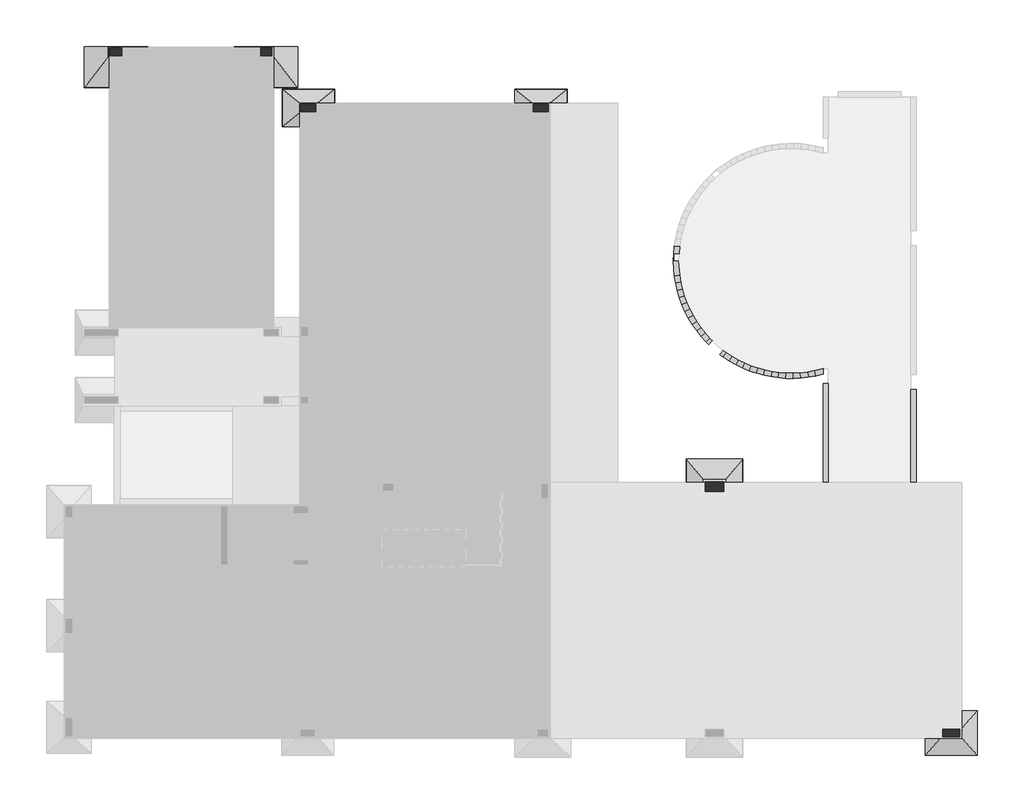
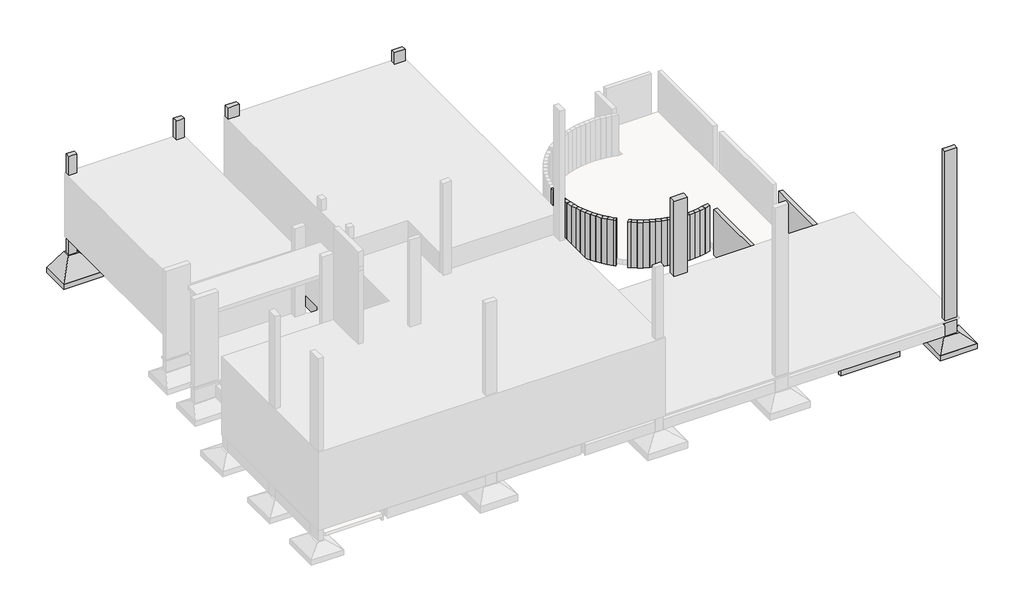
# One storey, part 3 of 4: 35 beams, 7 fasteners, 6 columns.
"""IFC4 building model written with IfcOpenShell, lengths in millimetres."""

import ifcopenshell
import ifcopenshell.guid

model = None  # the IFC model being written
_history = None  # IfcOwnerHistory: only IFC2X3 demands one
_inside = {}  # id of a spatial element -> (the spatial element, [elements in it])
_under = {}  # id of a project, library or spatial element -> (it, [spatial elements below it])
_declared = {}  # id of a project -> (the project, [libraries it declares])
_typed = {}  # id of a type object -> (the type object, [elements of that type])
_made_of = {}  # id of a material, layer set ... -> (it, [elements and type objects made of it])


def new_model(schema):
    """Start an empty IFC model of exactly this schema.

    Asked for "IFC4X3", IfcOpenShell would pick the latest addendum, in which some entities
    have other attributes; the version numbers below select the first issue.
    IFC2X3 requires an IfcOwnerHistory on every rooted entity: one is made here for all.
    """
    global model, _history
    if schema == "IFC4X3":
        model = ifcopenshell.file(schema_version=(4, 3, 0, 0))
    else:
        model = ifcopenshell.file(schema=schema)
    _inside.clear()
    _under.clear()
    _declared.clear()
    _typed.clear()
    _made_of.clear()
    _history = None
    if model.schema == "IFC2X3":
        org = make("IfcOrganization", Name="unknown")
        user = make(
            "IfcPersonAndOrganization",
            ThePerson=make("IfcPerson", FamilyName="unknown"),
            TheOrganization=org,
        )
        app = make(
            "IfcApplication",
            ApplicationDeveloper=org,
            Version="unknown",
            ApplicationFullName="unknown",
            ApplicationIdentifier="unknown",
        )
        _history = make(
            "IfcOwnerHistory",
            OwningUser=user,
            OwningApplication=app,
            ChangeAction="ADDED",
            CreationDate=0,
        )
    return model


def make(cls, **values):
    """One entity of the class cls with the attributes given. An attribute that is None is left unset."""
    return model.create_entity(
        cls, **{name: value for name, value in values.items() if value is not None}
    )


def rooted(cls, **values):
    """An entity with a GlobalId (a new one), such as an element, a storey or a relation."""
    return make(cls, GlobalId=ifcopenshell.guid.new(), OwnerHistory=_history, **values)


def si_unit(unit_type, name, prefix=None):
    """IfcSIUnit, for example si_unit("LENGTHUNIT", "METRE", prefix="MILLI")."""
    return make("IfcSIUnit", UnitType=unit_type, Prefix=prefix, Name=name)


def assignment(units):
    """IfcUnitAssignment: the units of a project."""
    return None if units is None else make("IfcUnitAssignment", Units=units)


def point(xyz):
    """IfcCartesianPoint."""
    return None if xyz is None else make("IfcCartesianPoint", Coordinates=xyz)


def direction(xyz):
    """IfcDirection."""
    return None if xyz is None else make("IfcDirection", DirectionRatios=xyz)


def frame(location, z_axis=None, x_axis=None):
    """IfcAxis2Placement3D, a coordinate frame: its origin and axes. An axis left out is left unset."""
    return make(
        "IfcAxis2Placement3D",
        Location=point(location),
        Axis=direction(z_axis),
        RefDirection=direction(x_axis),
    )


def frame_2d(location, x_axis=None):
    """IfcAxis2Placement2D, a coordinate frame in the plane: its origin and x axis."""
    return make(
        "IfcAxis2Placement2D", Location=point(location), RefDirection=direction(x_axis)
    )


def origin():
    """The frame at (0, 0, 0) with its axes left unset."""
    return frame((0.0, 0.0, 0.0))


def place(relative_to, where):
    """IfcLocalPlacement: puts the frame where relative to a parent placement (None: the world)."""
    return make(
        "IfcLocalPlacement", PlacementRelTo=relative_to, RelativePlacement=where
    )


def context(
    kind, dimensions, precision=None, world=None, true_north=None, identifier=None
):
    """IfcGeometricRepresentationContext, for example the 3D "Model" context."""
    return make(
        "IfcGeometricRepresentationContext",
        ContextIdentifier=identifier,
        ContextType=kind,
        CoordinateSpaceDimension=dimensions,
        Precision=precision,
        WorldCoordinateSystem=world,
        TrueNorth=true_north,
    )


def project(units=None, contexts=None):
    """IfcProject with its units and contexts."""
    return rooted(
        "IfcProject",
        Name="project",
        RepresentationContexts=contexts,
        UnitsInContext=assignment(units),
    )


def spatial(cls, under=None, at=None, **own):
    """A site, building, storey or space (cls), placed at a placement, below another one or the project."""
    s = rooted(cls, ObjectPlacement=at, **own)
    if under is not None:
        _under.setdefault(under.id(), (under, []))[1].append(s)
    return s


def polyline(points):
    """IfcPolyline through the points."""
    return make("IfcPolyline", Points=[point(p) for p in points])


def circle_curve(where, radius):
    """IfcCircle in the frame where."""
    return make("IfcCircle", Position=where, Radius=radius)


def trimmed(basis, trim1, trim2, sense, master):
    """IfcTrimmedCurve: the piece of a basis curve between two trims."""
    return make(
        "IfcTrimmedCurve",
        BasisCurve=basis,
        Trim1=trim1,
        Trim2=trim2,
        SenseAgreement=sense,
        MasterRepresentation=master,
    )


def segment(curve, same_sense, transition):
    """IfcCompositeCurveSegment."""
    return make(
        "IfcCompositeCurveSegment",
        Transition=transition,
        SameSense=same_sense,
        ParentCurve=curve,
    )


def composite_curve(segments, self_intersect=None):
    """IfcCompositeCurve: segments joined end to end."""
    return make("IfcCompositeCurve", Segments=segments, SelfIntersect=self_intersect)


def outline(outer, holes=None, kind="AREA"):
    """IfcArbitraryClosedProfileDef: a profile drawn as a closed curve; with holes, ...WithVoids."""
    if holes is None:
        return make("IfcArbitraryClosedProfileDef", ProfileType=kind, OuterCurve=outer)
    return make(
        "IfcArbitraryProfileDefWithVoids",
        ProfileType=kind,
        OuterCurve=outer,
        InnerCurves=holes,
    )


def extrude(swept, where, along, depth):
    """IfcExtrudedAreaSolid: the profile swept, set in the frame where, extruded along a direction by depth."""
    return make(
        "IfcExtrudedAreaSolid",
        SweptArea=swept,
        Position=where,
        ExtrudedDirection=direction(along),
        Depth=depth,
    )


def faces_of(points, faces, orient=None, outer=None):
    """IfcFace entities. A face is a list of loops; a loop is a list of indices into points, from 0.

    orient and outer hold one flag for each loop. By default every Orientation is true, the
    first loop of a face is its IfcFaceOuterBound and the others are IfcFaceBound.
    """
    made = []
    for i, loops in enumerate(faces):
        bounds = []
        for j, loop in enumerate(loops):
            is_outer = j == 0 if outer is None else outer[i][j]
            bounds.append(
                make(
                    "IfcFaceOuterBound" if is_outer else "IfcFaceBound",
                    Bound=make("IfcPolyLoop", Polygon=[points[k] for k in loop]),
                    Orientation=True if orient is None else orient[i][j],
                )
            )
        made.append(make("IfcFace", Bounds=bounds))
    return made


def faceted_brep(points, faces, orient=None, outer=None, voids=None):
    """IfcFacetedBrep: a solid bounded by flat faces; with voids (closed shells), ...WithVoids."""
    shared = [point(p) for p in points]
    hull = make("IfcClosedShell", CfsFaces=faces_of(shared, faces, orient, outer))
    if voids is None:
        return make("IfcFacetedBrep", Outer=hull)
    return make(
        "IfcFacetedBrepWithVoids",
        Outer=hull,
        Voids=[
            make(cls, CfsFaces=faces_of(shared, fs, o, b)) for cls, fs, o, b in voids
        ],
    )


def shape(context_of_items, identifier, shape_type, items):
    """IfcShapeRepresentation: the items that make up one representation, for example the "Body"."""
    return make(
        "IfcShapeRepresentation",
        ContextOfItems=context_of_items,
        RepresentationIdentifier=identifier,
        RepresentationType=shape_type,
        Items=items,
    )


def source(mapping_origin, context_of_items, identifier, shape_type, items):
    """IfcRepresentationMap: a shape defined once, which mapped items show again and again."""
    return make(
        "IfcRepresentationMap",
        MappingOrigin=mapping_origin,
        MappedRepresentation=shape(context_of_items, identifier, shape_type, items),
    )


def transform(
    local_origin,
    x_axis=None,
    y_axis=None,
    z_axis=None,
    scale=None,
    scale2=None,
    scale3=None,
    uniform=True,
):
    """IfcCartesianTransformationOperator3D, or its non-uniform kind. x_axis, y_axis, z_axis: its Axis1, 2, 3."""
    if uniform:
        return make(
            "IfcCartesianTransformationOperator3D",
            Axis1=direction(x_axis),
            Axis2=direction(y_axis),
            LocalOrigin=point(local_origin),
            Scale=scale,
            Axis3=direction(z_axis),
        )
    return make(
        "IfcCartesianTransformationOperator3DnonUniform",
        Axis1=direction(x_axis),
        Axis2=direction(y_axis),
        LocalOrigin=point(local_origin),
        Scale=scale,
        Axis3=direction(z_axis),
        Scale2=scale2,
        Scale3=scale3,
    )


def mapped(mapping_source, mapping_target):
    """IfcMappedItem: shows the shape of a source again, moved by a transform."""
    return make(
        "IfcMappedItem", MappingSource=mapping_source, MappingTarget=mapping_target
    )


def made_of(thing, what):
    """Note that an element or type object is made of a material, layer set ...; save() writes the relation."""
    if what is not None:
        _made_of.setdefault(what.id(), (what, []))[1].append(thing)
    return thing


def element(
    cls,
    number,
    at=None,
    inside=None,
    cuts=None,
    type_object=None,
    material=None,
    context=None,
    identifier="Body",
    shape_type=None,
    held_by="IfcProductDefinitionShape",
    body=None,
    shapes=None,
    **own,
):
    """One element of the class cls, such as IfcWall. Its Tag is "e" and its number.

    at: its placement. inside: the storey or other place that contains it. cuts: it is an
    opening in that element (IfcRelVoidsElement). A single representation is given by context,
    identifier, shape_type and body (its items); several are given by shapes. held_by: the class
    of the entity that holds the representations. save() writes the other relations.
    """
    e = rooted(cls, Tag="e%d" % number, ObjectPlacement=at, **own)
    if body is not None:
        shapes = [shape(context, identifier, shape_type, body)]
    if shapes is not None:
        e.Representation = make(held_by, Representations=shapes)
    if inside is not None:
        _inside.setdefault(inside.id(), (inside, []))[1].append(e)
    if cuts is not None:
        rooted(
            "IfcRelVoidsElement", RelatingBuildingElement=cuts, RelatedOpeningElement=e
        )
    if type_object is not None:
        _typed.setdefault(type_object.id(), (type_object, []))[1].append(e)
    return made_of(e, material)


def aggregate(whole, parts):
    """IfcRelAggregates: a whole, such as a stair, and the parts it consists of."""
    return rooted("IfcRelAggregates", RelatingObject=whole, RelatedObjects=parts)


def save(model, path):
    """Write the relations noted so far, then the file.

    IfcRelAggregates (storeys below a building ...), IfcRelContainedInSpatialStructure (elements
    in a storey), IfcRelDefinesByType, IfcRelAssociatesMaterial and IfcRelDeclares: one each for
    every whole, place, type object, material and project.
    """
    for whole, parts in _under.values():
        aggregate(whole, parts)
    for where, things in _inside.values():
        rooted(
            "IfcRelContainedInSpatialStructure",
            RelatedElements=things,
            RelatingStructure=where,
        )
    for kind, things in _typed.values():
        rooted("IfcRelDefinesByType", RelatedObjects=things, RelatingType=kind)
    for what, things in _made_of.values():
        rooted("IfcRelAssociatesMaterial", RelatedObjects=things, RelatingMaterial=what)
    for by, libraries in _declared.values():
        rooted("IfcRelDeclares", RelatingContext=by, RelatedDefinitions=libraries)
    model.write(path)


def tqs_viga_retangular_19_0_x_30_0_29604a85(model_context):
    return source(origin(), model_context, "Body", "SweptSolid", [
        extrude(outline(polyline([(1809.0, 95.0), (1809.0, -95.0), (-1809.0, -95.0), (-1809.0, 95.0), (1809.0, 95.0)])), frame((0.0, 0.0, -150.0), z_axis=(0.0, 0.0, 1.0), x_axis=(1.0, 0.0, 0.0)), (0.0, 0.0, 1.0), 300.0),
    ])


def s1_ccae0304(model_context):
    return source(origin(), model_context, "Body", "SolidModel", [
        faceted_brep([(-460.0, 0.0, 0.0), (-750.0, 0.0, 0.0), (-750.0, -400.0, 0.0), (-460.0, -400.0, 0.0), (350.0, 650.0, -400.0), (350.0, -1050.0, -400.0), (-750.0, -1050.0, -400.0), (-750.0, 650.0, -400.0)], [[[0, 1, 2, 3]], [[4, 5, 6, 7]], [[4, 7, 1, 0]], [[7, 6, 2, 1]], [[6, 5, 3, 2]], [[5, 4, 0, 3]]]),
        extrude(outline(polyline([(350.0, 650.0), (350.0, -1050.0), (-750.0, -1050.0), (-750.0, 650.0), (350.0, 650.0)])), frame((0.0, 0.0, -600.0), z_axis=(0.0, 0.0, 1.0), x_axis=(1.0, 0.0, 0.0)), (0.0, 0.0, 1.0), 200.0),
    ])


def s12_1e6d1b45(model_context):
    return source(origin(), model_context, "Body", "SolidModel", [
        faceted_brep([(-55.0, 50.0, 0.0), (-345.0, 50.0, 0.0), (-345.0, -450.0, 0.0), (-55.0, -450.0, 0.0), (550.0, 550.0, -350.0), (550.0, -950.0, -350.0), (-950.0, -950.0, -350.0), (-950.0, 550.0, -350.0)], [[[0, 1, 2, 3]], [[4, 5, 6, 7]], [[4, 7, 1, 0]], [[7, 6, 2, 1]], [[6, 5, 3, 2]], [[5, 4, 0, 3]]]),
        extrude(outline(polyline([(550.0, 550.0), (550.0, -950.0), (-950.0, -950.0), (-950.0, 550.0), (550.0, 550.0)])), frame((0.0, 0.0, -600.0), z_axis=(0.0, 0.0, 1.0), x_axis=(1.0, 0.0, 0.0)), (0.0, 0.0, 1.0), 250.0),
    ])


def s13_7eae1afe(model_context):
    return source(origin(), model_context, "Body", "SolidModel", [
        faceted_brep([(-5.0, 100.0, 0.0), (-395.0, 100.0, 0.0), (-395.0, -500.0, 0.0), (-5.0, -500.0, 0.0), (550.0, 550.0, -300.0), (550.0, -950.0, -300.0), (-950.0, -950.0, -300.0), (-950.0, 550.0, -300.0)], [[[0, 1, 2, 3]], [[4, 5, 6, 7]], [[4, 7, 1, 0]], [[7, 6, 2, 1]], [[6, 5, 3, 2]], [[5, 4, 0, 3]]]),
        extrude(outline(polyline([(550.0, 550.0), (550.0, -950.0), (-950.0, -950.0), (-950.0, 550.0), (550.0, 550.0)])), frame((0.0, 0.0, -500.0), z_axis=(0.0, 0.0, 1.0), x_axis=(1.0, 0.0, 0.0)), (0.0, 0.0, 1.0), 200.0),
    ])


def s20_c409a0c5(model_context):
    return source(origin(), model_context, "Body", "SolidModel", [
        faceted_brep([(-55.0, 100.0, 0.0), (-345.0, 100.0, 0.0), (-345.0, -500.0, 0.0), (-55.0, -500.0, 0.0), (400.0, 500.0, -300.0), (400.0, -900.0, -300.0), (-800.0, -900.0, -300.0), (-800.0, 500.0, -300.0)], [[[0, 1, 2, 3]], [[4, 5, 6, 7]], [[4, 7, 1, 0]], [[7, 6, 2, 1]], [[6, 5, 3, 2]], [[5, 4, 0, 3]]]),
        extrude(outline(polyline([(400.0, 500.0), (400.0, -900.0), (-800.0, -900.0), (-800.0, 500.0), (400.0, 500.0)])), frame((0.0, 0.0, -500.0), z_axis=(0.0, 0.0, 1.0), x_axis=(1.0, 0.0, 0.0)), (0.0, 0.0, 1.0), 200.0),
    ])


def s3_fc183e28(model_context):
    return source(origin(), model_context, "Body", "SolidModel", [
        faceted_brep([(-55.0, 50.0, 0.0), (-345.0, 50.0, 0.0), (-345.0, -450.0, 0.0), (-55.0, -450.0, 0.0), (300.0, 500.0, -300.0), (300.0, -900.0, -300.0), (-700.0, -900.0, -300.0), (-700.0, 500.0, -300.0)], [[[0, 1, 2, 3]], [[4, 5, 6, 7]], [[4, 7, 1, 0]], [[7, 6, 2, 1]], [[6, 5, 3, 2]], [[5, 4, 0, 3]]]),
        extrude(outline(polyline([(300.0, 500.0), (300.0, -900.0), (-700.0, -900.0), (-700.0, 500.0), (300.0, 500.0)])), frame((0.0, 0.0, -500.0), z_axis=(0.0, 0.0, 1.0), x_axis=(1.0, 0.0, 0.0)), (0.0, 0.0, 1.0), 200.0),
    ])


model = new_model("IFC4")

# Units and contexts
model_context = context("Model", 3, world=origin())
ifc_project = project(units=[si_unit("LENGTHUNIT", "METRE", prefix="MILLI")], contexts=[model_context])

# Site, building, storey
site = spatial("IfcSite", under=ifc_project)
building = spatial("IfcBuilding", under=site)
storey = spatial("IfcBuildingStorey", under=building, Name="PAVIMENTO TÉRREO", Elevation=500.0)

# Beams
placement = place(None, origin())
element("IfcBeam", 1, ObjectType="TQS - Viga retangular : 14.0 x 180.0", at=placement, inside=storey, context=model_context, shape_type="Brep", body=[
    faceted_brep([(9682.718693, -9679.5699847, 350.0), (9682.718693, -9539.5699847, 350.0), (7474.718693, -9539.5699847, 350.0), (7474.718693, -9679.5699847, 350.0), (9682.718693, -9679.5699847, -1450.0), (7474.718693, -9679.5699847, -1450.0), (9682.718693, -9539.5699847, -1450.0), (7474.718693, -9539.5699847, -1450.0), (9682.718693, -9539.5699847, -1250.0), (7474.718693, -9539.5699847, -1250.0)], [[[0, 1, 2, 3]], [[4, 0, 3, 5]], [[6, 4, 5, 7]], [[1, 8, 6, 7, 9, 2]], [[2, 9, 7, 5, 3]], [[1, 0, 4, 6, 8]]]),
])
element("IfcBeam", 2, ObjectType="TQS - Viga retangular : 14.0 x 180.0", at=placement, inside=storey, context=model_context, shape_type="Brep", body=[
    faceted_brep([(7474.718693, -1696.0936198, 350.0), (7334.718693, -1696.0936198, 350.0), (7334.718693, -5230.1494451, 350.0), (7474.718693, -5230.1494451, 350.0), (7474.718693, -5230.1494451, -1250.0), (7474.718693, -5230.1494451, -1450.0), (7474.718693, -1696.0936198, -1450.0), (7474.718693, -1696.0936198, -1250.0), (7334.718693, -1696.0936198, -1450.0), (7334.718693, -5230.1494451, -1450.0)], [[[0, 1, 2, 3]], [[0, 3, 4, 5, 6, 7]], [[8, 6, 5, 9]], [[1, 8, 9, 2]], [[1, 0, 7, 6, 8]], [[3, 2, 9, 5, 4]]]),
    faceted_brep([(7334.718693, -5630.1494451, 350.0), (7474.718693, -5630.1494451, 350.0), (7474.718693, -5630.1494451, -1250.0), (7474.718693, -5630.1494451, -1450.0), (7334.718693, -5630.1494451, -1450.0), (7334.718693, -9279.5699847, 350.0), (7474.718693, -9279.5699847, 350.0), (7474.718693, -9279.5699847, -1250.0), (7474.718693, -9279.5699847, -1450.0), (7334.718693, -9279.5699847, -1450.0)], [[[0, 1, 2, 3, 4]], [[1, 0, 5, 6]], [[1, 6, 7, 8, 3, 2]], [[4, 3, 8, 9]], [[0, 4, 9, 5]], [[6, 5, 9, 8, 7]]]),
])
element("IfcBeam", 3, ObjectType="TQS - Viga retangular : 14.0 x 180.0", at=placement, inside=storey, context=model_context, shape_type="Brep", body=[
    faceted_brep([(7334.718693, -1296.0936198, 350.0), (7106.1277936, -1352.3610531, 350.0), (7135.2990206, -1489.35947, 350.0), (7334.718693, -1440.2725066, 350.0), (7334.718693, -1296.0936198, -1250.0), (7334.718693, -1296.0936198, -1450.0), (7106.1277936, -1352.3610531, -1450.0), (7106.1277936, -1352.3610531, -1250.0), (7334.718693, -1440.2725066, -1450.0), (7135.2990206, -1489.35947, -1450.0)], [[[0, 1, 2, 3]], [[1, 0, 4, 5, 6, 7]], [[6, 5, 8, 9]], [[3, 2, 9, 8]], [[0, 3, 8, 5, 4]], [[2, 1, 7, 6, 9]]]),
])
element("IfcBeam", 4, ObjectType="TQS - Viga retangular : 14.0 x 180.0", at=placement, inside=storey, context=model_context, shape_type="Brep", body=[
    faceted_brep([(6938.2242767, -1524.8638101, 350.0), (7135.2990206, -1489.35947, 350.0), (7106.1277936, -1352.3610531, 350.0), (6917.7849868, -1386.2922761, 350.0), (7106.1277936, -1352.3610531, -1250.0), (7106.1277936, -1352.3610531, -1450.0), (6917.7849868, -1386.2922761, -1450.0), (6917.7849868, -1386.2922761, -1250.0), (7135.2990206, -1489.35947, -1450.0), (6938.2242767, -1524.8638101, -1450.0)], [[[0, 1, 2, 3]], [[3, 2, 4, 5, 6, 7]], [[6, 5, 8, 9]], [[1, 0, 9, 8]], [[1, 8, 5, 4, 2]], [[0, 3, 7, 6, 9]]]),
])
element("IfcBeam", 5, ObjectType="TQS - Viga retangular : 14.0 x 180.0", at=placement, inside=storey, context=model_context, shape_type="Brep", body=[
    faceted_brep([(6739.2913899, -1547.770563, 350.0), (6938.2242767, -1524.8638101, 350.0), (6917.7849868, -1386.2922761, 350.0), (6727.7008432, -1408.1801126, 350.0), (6917.7849868, -1386.2922761, -1250.0), (6917.7849868, -1386.2922761, -1450.0), (6727.7008432, -1408.1801126, -1450.0), (6727.7008432, -1408.1801126, -1250.0), (6938.2242767, -1524.8638101, -1450.0), (6739.2913899, -1547.770563, -1450.0)], [[[0, 1, 2, 3]], [[3, 2, 4, 5, 6, 7]], [[6, 5, 8, 9]], [[1, 0, 9, 8]], [[1, 8, 5, 4, 2]], [[0, 3, 7, 6, 9]]]),
])
element("IfcBeam", 6, ObjectType="TQS - Viga retangular : 14.0 x 180.0", at=placement, inside=storey, context=model_context, shape_type="Brep", body=[
    faceted_brep([(6539.3048029, -1557.9870986, 350.0), (6739.2913899, -1547.770563, 350.0), (6727.7008432, -1408.1801126, 350.0), (6536.6098693, -1417.942206, 350.0), (6727.7008432, -1408.1801126, -1250.0), (6727.7008432, -1408.1801126, -1450.0), (6536.6098693, -1417.942206, -1450.0), (6536.6098693, -1417.942206, -1250.0), (6739.2913899, -1547.770563, -1450.0), (6539.3048029, -1557.9870986, -1450.0)], [[[0, 1, 2, 3]], [[3, 2, 4, 5, 6, 7]], [[6, 5, 8, 9]], [[1, 0, 9, 8]], [[1, 8, 5, 4, 2]], [[0, 3, 7, 6, 9]]]),
])
element("IfcBeam", 7, ObjectType="TQS - Viga retangular : 14.0 x 180.0", at=placement, inside=storey, context=model_context, shape_type="Brep", body=[
    faceted_brep([(6339.0732182, -1555.4721035, 350.0), (6539.3048029, -1557.9870986, 350.0), (6536.6098693, -1417.942206, 350.0), (6345.2847953, -1415.5390805, 350.0), (6536.6098693, -1417.942206, -1250.0), (6536.6098693, -1417.942206, -1450.0), (6345.2847953, -1415.5390805, -1450.0), (6345.2847953, -1415.5390805, -1250.0), (6539.3048029, -1557.9870986, -1450.0), (6339.0732182, -1555.4721035, -1450.0)], [[[0, 1, 2, 3]], [[3, 2, 4, 5, 6, 7]], [[6, 5, 8, 9]], [[1, 0, 9, 8]], [[1, 8, 5, 4, 2]], [[0, 3, 7, 6, 9]]]),
])
element("IfcBeam", 8, ObjectType="TQS - Viga retangular : 14.0 x 180.0", at=placement, inside=storey, context=model_context, shape_type="Brep", body=[
    faceted_brep([(6139.4063301, -1540.2357477, 350.0), (6339.0732182, -1555.4721035, 350.0), (6345.2847953, -1415.5390805, 350.0), (6154.4732894, -1400.978469, 350.0), (6345.2847953, -1415.5390805, -1250.0), (6345.2847953, -1415.5390805, -1450.0), (6154.4732894, -1400.978469, -1450.0), (6154.4732894, -1400.978469, -1250.0), (6339.0732182, -1555.4721035, -1450.0), (6139.4063301, -1540.2357477, -1450.0)], [[[0, 1, 2, 3]], [[3, 2, 4, 5, 6, 7]], [[6, 5, 8, 9]], [[1, 0, 9, 8]], [[1, 8, 5, 4, 2]], [[0, 3, 7, 6, 9]]]),
])
element("IfcBeam", 9, ObjectType="TQS - Viga retangular : 14.0 x 180.0", at=placement, inside=storey, context=model_context, shape_type="Brep", body=[
    faceted_brep([(5942.253541, -1512.5751442, 350.0), (6139.4063301, -1540.2357477, 350.0), (6154.4732894, -1400.978469, 350.0), (5966.1413215, -1374.5554297, 350.0), (6154.4732894, -1400.978469, -1250.0), (6154.4732894, -1400.978469, -1450.0), (5966.1413215, -1374.5554297, -1450.0), (5966.1413215, -1374.5554297, -1250.0), (6139.4063301, -1540.2357477, -1450.0), (5942.253541, -1512.5751442, -1450.0)], [[[0, 1, 2, 3]], [[3, 2, 4, 5, 6, 7]], [[6, 5, 8, 9]], [[1, 0, 9, 8]], [[1, 8, 5, 4, 2]], [[0, 3, 7, 6, 9]]]),
])
element("IfcBeam", 10, ObjectType="TQS - Viga retangular : 14.0 x 180.0", at=placement, inside=storey, context=model_context, shape_type="Brep", body=[
    faceted_brep([(5746.1327296, -1472.1320983, 350.0), (5942.253541, -1512.5751442, 350.0), (5966.1413215, -1374.5554297, 350.0), (5778.7697179, -1335.9166013, 350.0), (5966.1413215, -1374.5554297, -1250.0), (5966.1413215, -1374.5554297, -1450.0), (5778.7697179, -1335.9166013, -1450.0), (5778.7697179, -1335.9166013, -1250.0), (5942.253541, -1512.5751442, -1450.0), (5746.1327296, -1472.1320983, -1450.0)], [[[0, 1, 2, 3]], [[3, 2, 4, 5, 6, 7]], [[6, 5, 8, 9]], [[1, 0, 9, 8]], [[1, 8, 5, 4, 2]], [[0, 3, 7, 6, 9]]]),
])
element("IfcBeam", 11, ObjectType="TQS - Viga retangular : 14.0 x 180.0", at=placement, inside=storey, context=model_context, shape_type="Brep", body=[
    faceted_brep([(5552.9789583, -1419.3056534, 350.0), (5746.1327296, -1472.1320983, 350.0), (5778.7697179, -1335.9166013, 350.0), (5594.2076289, -1285.4399321, 350.0), (5778.7697179, -1335.9166013, -1250.0), (5778.7697179, -1335.9166013, -1450.0), (5594.2076289, -1285.4399321, -1450.0), (5594.2076289, -1285.4399321, -1250.0), (5746.1327296, -1472.1320983, -1450.0), (5552.9789583, -1419.3056534, -1450.0)], [[[0, 1, 2, 3]], [[3, 2, 4, 5, 6, 7]], [[6, 5, 8, 9]], [[1, 0, 9, 8]], [[1, 8, 5, 4, 2]], [[0, 3, 7, 6, 9]]]),
])
element("IfcBeam", 12, ObjectType="TQS - Viga retangular : 14.0 x 180.0", at=placement, inside=storey, context=model_context, shape_type="Brep", body=[
    faceted_brep([(5363.9986658, -1354.4553965, 350.0), (5552.9789583, -1419.3056534, 350.0), (5594.2076289, -1285.4399321, 350.0), (5413.6522985, -1223.4807754, 350.0), (5594.2076289, -1285.4399321, -1250.0), (5594.2076289, -1285.4399321, -1450.0), (5413.6522985, -1223.4807754, -1450.0), (5413.6522985, -1223.4807754, -1250.0), (5552.9789583, -1419.3056534, -1450.0), (5363.9986658, -1354.4553965, -1450.0)], [[[0, 1, 2, 3]], [[3, 2, 4, 5, 6, 7]], [[6, 5, 8, 9]], [[1, 0, 9, 8]], [[1, 8, 5, 4, 2]], [[0, 3, 7, 6, 9]]]),
])
element("IfcBeam", 13, ObjectType="TQS - Viga retangular : 14.0 x 180.0", at=placement, inside=storey, context=model_context, shape_type="Brep", body=[
    faceted_brep([(5179.1069104, -1277.5521698, 350.0), (5363.9986658, -1354.4553965, 350.0), (5413.6522985, -1223.4807754, 350.0), (5236.9847165, -1149.9982825, 350.0), (5413.6522985, -1223.4807754, -1250.0), (5413.6522985, -1223.4807754, -1450.0), (5236.9847165, -1149.9982825, -1450.0), (5236.9847165, -1149.9982825, -1250.0), (5363.9986658, -1354.4553965, -1450.0), (5179.1069104, -1277.5521698, -1450.0)], [[[0, 1, 2, 3]], [[3, 2, 4, 5, 6, 7]], [[6, 5, 8, 9]], [[1, 0, 9, 8]], [[1, 8, 5, 4, 2]], [[0, 3, 7, 6, 9]]]),
])
element("IfcBeam", 14, ObjectType="TQS - Viga retangular : 14.0 x 180.0", at=placement, inside=storey, context=model_context, shape_type="Brep", body=[
    faceted_brep([(4999.4769736, -1189.0530269, 350.0), (5179.1069104, -1277.5521698, 350.0), (5236.9847165, -1149.9982825, 350.0), (5065.344906, -1065.4356735, 350.0), (5236.9847165, -1149.9982825, -1250.0), (5236.9847165, -1149.9982825, -1450.0), (5065.344906, -1065.4356735, -1450.0), (5065.344906, -1065.4356735, -1250.0), (5179.1069104, -1277.5521698, -1450.0), (4999.4769736, -1189.0530269, -1450.0)], [[[0, 1, 2, 3]], [[3, 2, 4, 5, 6, 7]], [[6, 5, 8, 9]], [[1, 0, 9, 8]], [[1, 8, 5, 4, 2]], [[0, 3, 7, 6, 9]]]),
])
element("IfcBeam", 15, ObjectType="TQS - Viga retangular : 14.0 x 180.0", at=placement, inside=storey, context=model_context, shape_type="Brep", body=[
    faceted_brep([(4825.8347061, -1089.3155581, 350.0), (4999.4769736, -1189.0530269, 350.0), (5065.344906, -1065.4356735, 350.0), (4899.4264221, -970.1346281, 350.0), (5065.344906, -1065.4356735, -1250.0), (5065.344906, -1065.4356735, -1450.0), (4899.4264221, -970.1346281, -1450.0), (4899.4264221, -970.1346281, -1250.0), (4999.4769736, -1189.0530269, -1450.0), (4825.8347061, -1089.3155581, -1450.0)], [[[0, 1, 2, 3]], [[3, 2, 4, 5, 6, 7]], [[6, 5, 8, 9]], [[1, 0, 9, 8]], [[1, 8, 5, 4, 2]], [[0, 3, 7, 6, 9]]]),
])
element("IfcBeam", 16, ObjectType="TQS - Viga retangular : 14.0 x 180.0", at=placement, inside=storey, context=model_context, shape_type="Brep", body=[
    faceted_brep([(4659.7082838, -979.2900143, 350.0), (4825.8347061, -1089.3155581, 350.0), (4899.4264221, -970.1346281, 350.0), (4740.8701617, -865.1228032, 350.0), (4899.4264221, -970.1346281, -1250.0), (4899.4264221, -970.1346281, -1450.0), (4740.8701617, -865.1228032, -1450.0), (4740.8701617, -865.1228032, -1250.0), (4825.8347061, -1089.3155581, -1450.0), (4659.7082838, -979.2900143, -1450.0)], [[[0, 1, 2, 3]], [[3, 2, 4, 5, 6, 7]], [[6, 5, 8, 9]], [[1, 0, 9, 8]], [[1, 8, 5, 4, 2]], [[0, 3, 7, 6, 9]]]),
])
element("IfcBeam", 17, ObjectType="TQS - Viga retangular : 14.0 x 180.0", at=placement, inside=storey, context=model_context, shape_type="Brep", body=[
    faceted_brep([(4571.9800682, -912.4546637, 350.0), (4659.7082838, -979.2900143, 350.0), (4740.8701617, -865.1228032, 350.0), (4665.976342, -808.0652799, 350.0), (4740.8701617, -865.1228032, -1250.0), (4740.8701617, -865.1228032, -1450.0), (4665.976342, -808.0652799, -1450.0), (4665.976342, -808.0652799, -1250.0), (4659.7082838, -979.2900143, -1450.0), (4571.9800682, -912.4546637, -1450.0)], [[[0, 1, 2, 3]], [[3, 2, 4, 5, 6, 7]], [[8, 9, 6, 5]], [[1, 0, 9, 8]], [[0, 3, 7, 6, 9]], [[1, 8, 5, 4, 2]]]),
])
element("IfcBeam", 18, ObjectType="TQS - Viga retangular : 14.0 x 180.0", at=placement, inside=storey, context=model_context, shape_type="Brep", body=[
    faceted_brep([(4206.3905749, -587.9275531, 350.0), (4270.2869357, -650.1191423, 350.0), (4367.9344995, -549.7949015, 350.0), (4307.4254093, -490.9002096, 350.0), (4367.9344995, -549.7949015, -1450.0), (4362.9503182, -544.9436994, -1450.0), (4307.4254093, -490.9002096, -1450.0), (4307.4254093, -490.9002096, -1250.0), (4270.2869357, -650.1191423, -1450.0), (4206.3905749, -587.9275531, -1450.0)], [[[0, 1, 2, 3]], [[3, 2, 4, 5, 6, 7]], [[8, 9, 6, 5, 4]], [[1, 0, 9, 8]], [[1, 8, 4, 2]], [[0, 3, 7, 6, 9]]]),
])
element("IfcBeam", 19, ObjectType="TQS - Viga retangular : 14.0 x 180.0", at=placement, inside=storey, context=model_context, shape_type="Brep", body=[
    faceted_brep([(4072.6403676, -438.8977092, 350.0), (4206.3905749, -587.9275531, 350.0), (4307.4254093, -490.9002096, 350.0), (4179.8070625, -348.7027306, 350.0), (4307.4254093, -490.9002096, -1250.0), (4307.4254093, -490.9002096, -1450.0), (4179.8070625, -348.7027306, -1450.0), (4179.8070625, -348.7027306, -1250.0), (4206.3905749, -587.9275531, -1450.0), (4072.6403676, -438.8977092, -1450.0)], [[[0, 1, 2, 3]], [[3, 2, 4, 5, 6, 7]], [[6, 5, 8, 9]], [[1, 0, 9, 8]], [[1, 8, 5, 4, 2]], [[0, 3, 7, 6, 9]]]),
])
element("IfcBeam", 20, ObjectType="TQS - Viga retangular : 14.0 x 180.0", at=placement, inside=storey, context=model_context, shape_type="Brep", body=[
    faceted_brep([(3949.2502321, -282.451126, 350.0), (4072.6403676, -438.8977092, 350.0), (4179.8070625, -348.7027306, 350.0), (4061.9329165, -199.2498808, 350.0), (4179.8070625, -348.7027306, -1250.0), (4179.8070625, -348.7027306, -1450.0), (4061.9329165, -199.2498808, -1450.0), (4061.9329165, -199.2498808, -1250.0), (4072.6403676, -438.8977092, -1450.0), (3949.2502321, -282.451126, -1450.0)], [[[0, 1, 2, 3]], [[3, 2, 4, 5, 6, 7]], [[6, 5, 8, 9]], [[1, 0, 9, 8]], [[1, 8, 5, 4, 2]], [[0, 3, 7, 6, 9]]]),
])
element("IfcBeam", 21, ObjectType="TQS - Viga retangular : 14.0 x 180.0", at=placement, inside=storey, context=model_context, shape_type="Brep", body=[
    faceted_brep([(3835.4866089, -117.6577696, 350.0), (3949.2502321, -282.451126, 350.0), (4061.9329165, -199.2498808, 350.0), (3953.2296156, -41.7867013, 350.0), (4061.9329165, -199.2498808, -1250.0), (4061.9329165, -199.2498808, -1450.0), (3953.2296156, -41.7867013, -1450.0), (3953.2296156, -41.7867013, -1250.0), (3949.2502321, -282.451126, -1450.0), (3835.4866089, -117.6577696, -1450.0)], [[[0, 1, 2, 3]], [[3, 2, 4, 5, 6, 7]], [[6, 5, 8, 9]], [[1, 0, 9, 8]], [[1, 8, 5, 4, 2]], [[0, 3, 7, 6, 9]]]),
])
element("IfcBeam", 22, ObjectType="TQS - Viga retangular : 14.0 x 180.0", at=placement, inside=storey, context=model_context, shape_type="Brep", body=[
    faceted_brep([(3732.4270441, 54.0330523, 350.0), (3835.4866089, -117.6577696, 350.0), (3953.2296156, -41.7867013, 350.0), (3854.7542482, 122.2671329, 350.0), (3953.2296156, -41.7867013, -1250.0), (3953.2296156, -41.7867013, -1450.0), (3854.7542482, 122.2671329, -1450.0), (3854.7542482, 122.2671329, -1250.0), (3835.4866089, -117.6577696, -1450.0), (3732.4270441, 54.0330523, -1450.0)], [[[0, 1, 2, 3]], [[3, 2, 4, 5, 6, 7]], [[6, 5, 8, 9]], [[1, 0, 9, 8]], [[1, 8, 5, 4, 2]], [[0, 3, 7, 6, 9]]]),
])
element("IfcBeam", 23, ObjectType="TQS - Viga retangular : 14.0 x 180.0", at=placement, inside=storey, context=model_context, shape_type="Brep", body=[
    faceted_brep([(3640.48809, 231.9274426, 350.0), (3732.4270441, 54.0330523, 350.0), (3854.7542482, 122.2671329, 350.0), (3766.9048318, 292.2486007, 350.0), (3854.7542482, 122.2671329, -1250.0), (3854.7542482, 122.2671329, -1450.0), (3766.9048318, 292.2486007, -1450.0), (3766.9048318, 292.2486007, -1250.0), (3732.4270441, 54.0330523, -1450.0), (3640.48809, 231.9274426, -1450.0)], [[[0, 1, 2, 3]], [[3, 2, 4, 5, 6, 7]], [[6, 5, 8, 9]], [[1, 0, 9, 8]], [[1, 8, 5, 4, 2]], [[0, 3, 7, 6, 9]]]),
])
element("IfcBeam", 24, ObjectType="TQS - Viga retangular : 14.0 x 180.0", at=placement, inside=storey, context=model_context, shape_type="Brep", body=[
    faceted_brep([(3560.3661231, 414.5663391, 350.0), (3640.48809, 231.9274426, 350.0), (3766.9048318, 292.2486007, 350.0), (3690.3611932, 466.7306588, 350.0), (3766.9048318, 292.2486007, -1250.0), (3766.9048318, 292.2486007, -1450.0), (3690.3611932, 466.7306588, -1450.0), (3690.3611932, 466.7306588, -1250.0), (3640.48809, 231.9274426, -1450.0), (3560.3661231, 414.5663391, -1450.0)], [[[0, 1, 2, 3]], [[3, 2, 4, 5, 6, 7]], [[6, 5, 8, 9]], [[1, 0, 9, 8]], [[1, 8, 5, 4, 2]], [[0, 3, 7, 6, 9]]]),
])
element("IfcBeam", 25, ObjectType="TQS - Viga retangular : 14.0 x 180.0", at=placement, inside=storey, context=model_context, shape_type="Brep", body=[
    faceted_brep([(3491.737855, 602.6864416, 350.0), (3560.3661231, 414.5663391, 350.0), (3690.3611932, 466.7306588, 350.0), (3624.7902852, 646.4700908, 350.0), (3690.3611932, 466.7306588, -1250.0), (3690.3611932, 466.7306588, -1450.0), (3624.7902852, 646.4700908, -1450.0), (3624.7902852, 646.4700908, -1250.0), (3560.3661231, 414.5663391, -1450.0), (3491.737855, 602.6864416, -1450.0)], [[[0, 1, 2, 3]], [[3, 2, 4, 5, 6, 7]], [[6, 5, 8, 9]], [[1, 0, 9, 8]], [[1, 8, 5, 4, 2]], [[0, 3, 7, 6, 9]]]),
])
element("IfcBeam", 26, ObjectType="TQS - Viga retangular : 14.0 x 180.0", at=placement, inside=storey, context=model_context, shape_type="Brep", body=[
    faceted_brep([(3435.4159463, 794.2099051, 350.0), (3491.737855, 602.6864416, 350.0), (3624.7902852, 646.4700908, 350.0), (3570.9813422, 829.4481782, 350.0), (3624.7902852, 646.4700908, -1250.0), (3624.7902852, 646.4700908, -1450.0), (3570.9813422, 829.4481782, -1450.0), (3570.9813422, 829.4481782, -1250.0), (3491.737855, 602.6864416, -1450.0), (3435.4159463, 794.2099051, -1450.0)], [[[0, 1, 2, 3]], [[3, 2, 4, 5, 6, 7]], [[6, 5, 8, 9]], [[1, 0, 9, 8]], [[1, 8, 5, 4, 2]], [[0, 3, 7, 6, 9]]]),
])
element("IfcBeam", 27, ObjectType="TQS - Viga retangular : 14.0 x 180.0", at=placement, inside=storey, context=model_context, shape_type="Brep", body=[
    faceted_brep([(3391.2071159, 989.5163089, 350.0), (3435.4159463, 794.2099051, 350.0), (3570.9813422, 829.4481782, 350.0), (3528.735935, 1016.0805429, 350.0), (3570.9813422, 829.4481782, -1250.0), (3570.9813422, 829.4481782, -1450.0), (3528.735935, 1016.0805429, -1450.0), (3528.735935, 1016.0805429, -1250.0), (3435.4159463, 794.2099051, -1450.0), (3391.2071159, 989.5163089, -1450.0)], [[[0, 1, 2, 3]], [[3, 2, 4, 5, 6, 7]], [[6, 5, 8, 9]], [[1, 0, 9, 8]], [[1, 8, 5, 4, 2]], [[0, 3, 7, 6, 9]]]),
])
element("IfcBeam", 28, ObjectType="TQS - Viga retangular : 14.0 x 180.0", at=placement, inside=storey, context=model_context, shape_type="Brep", body=[
    faceted_brep([(3359.6001228, 1186.6200486, 350.0), (3391.2071159, 989.5163089, 350.0), (3528.735935, 1016.0805429, 350.0), (3498.5672214, 1204.2150568, 350.0), (3528.735935, 1016.0805429, -1250.0), (3528.735935, 1016.0805429, -1450.0), (3498.5672214, 1204.2150568, -1450.0), (3498.5672214, 1204.2150568, -1250.0), (3391.2071159, 989.5163089, -1450.0), (3359.6001228, 1186.6200486, -1450.0)], [[[0, 1, 2, 3]], [[3, 2, 4, 5, 6, 7]], [[6, 5, 8, 9]], [[1, 0, 9, 8]], [[1, 8, 5, 4, 2]], [[0, 3, 7, 6, 9]]]),
])
element("IfcBeam", 29, ObjectType="TQS - Viga retangular : 14.0 x 180.0", at=placement, inside=storey, context=model_context, shape_type="Brep", body=[
    faceted_brep([(3322.4683621, 1585.2441839, 350.0), (3359.6001228, 1186.6200486, 350.0), (3498.5672214, 1204.2150568, 350.0), (3463.0733079, 1585.2562551, 350.0), (3335.9283808, 1585.2453395, 350.0), (3498.5672214, 1204.2150568, -1250.0), (3498.5672214, 1204.2150568, -1450.0), (3481.6870042, 1385.4308636, -1450.0), (3463.0733079, 1585.2562551, -1450.0), (3359.6001228, 1186.6200486, -1450.0), (3322.4683621, 1585.2441839, -1450.0), (3335.9283808, 1585.2453395, -1450.0)], [[[0, 1, 2, 3, 4]], [[3, 2, 5, 6, 7, 8]], [[9, 10, 11, 8, 7, 6]], [[1, 0, 10, 9]], [[0, 4, 3, 8, 11, 10]], [[1, 9, 6, 5, 2]]]),
])
element("IfcBeam", 30, ObjectType="TQS - Viga retangular : 14.0 x 180.0", at=placement, inside=storey, context=model_context, shape_type="SweptSolid", body=[
    extrude(outline(polyline([(3322.4683621, 1585.2441839), (3359.6197005, 1984.821412), (3498.5878389, 1967.228978), (3481.5501681, 1783.9821402), (3342.1096921, 1786.0821852), (3335.8794834, 1590.2360081), (3335.9283808, 1585.2453395), (3322.4683621, 1585.2441839)])), frame((0.0, 0.0, -1450.0), z_axis=(0.0, 0.0, 1.0), x_axis=(1.0, 0.0, 0.0)), (0.0, 0.0, 1.0), 1800.0),
])
element("IfcBeam", 31, ObjectType="TQS - Viga retangular : 14.0 x 180.0", at=placement, inside=storey, context=model_context, shape_type="SweptSolid", body=[
    extrude(outline(polyline([(9822.718693, -5230.1494451), (9682.718693, -5230.1494451), (9682.718693, -1851.4011146), (9822.718693, -1851.4011146), (9822.718693, -5230.1494451)])), frame((0.0, 0.0, -1450.0), z_axis=(0.0, 0.0, 1.0), x_axis=(1.0, 0.0, 0.0)), (0.0, 0.0, 1.0), 1800.0),
    extrude(outline(polyline([(9822.718693, -9279.5699847), (9682.718693, -9279.5699847), (9682.718693, -5630.1494451), (9822.718693, -5630.1494451), (9822.718693, -9279.5699847)])), frame((0.0, 0.0, -1450.0), z_axis=(0.0, 0.0, 1.0), x_axis=(1.0, 0.0, 0.0)), (0.0, 0.0, 1.0), 1800.0),
])
tqs_viga_retangular_19_0_x_30_0_shape = tqs_viga_retangular_19_0_x_30_0_29604a85(model_context)
element("IfcBeam", 32, ObjectType="TQS - Viga retangular : 19.0 x 30.0", at=placement, inside=storey, context=model_context, shape_type="MappedRepresentation", body=[
    mapped(tqs_viga_retangular_19_0_x_30_0_shape, transform((-9571.281307, 7179.4300153, 50.0), x_axis=(1.0, 0.0, 0.0), y_axis=(0.0, 1.0, 0.0), z_axis=(0.0, 0.0, 1.0))),
])
element("IfcBeam", 33, ObjectType="TQS - Viga retangular : 19.0 x 40.0", at=placement, inside=storey, context=model_context, shape_type="SweptSolid", body=[
    extrude(outline(composite_curve([segment(polyline([(-412.281307, 5774.4300153), (-412.281307, 5584.4300153), (-3240.0409229, 5584.4300153)]), True, "CONTINUOUS"), segment(trimmed(circle_curve(frame_2d((-3321.281307, 5679.4300153)), 125.0), [point((-3240.0409229, 5584.4300153))], [point((-3196.281307, 5679.4300153))], True, "CARTESIAN"), True, "CONTINUOUS"), segment(trimmed(circle_curve(frame_2d((-3321.281307, 5679.4300153)), 125.0), [point((-3196.281307, 5679.4300153))], [point((-3240.0409229, 5774.4300153))], True, "CARTESIAN"), True, "CONTINUOUS"), segment(polyline([(-3240.0409229, 5774.4300153), (-412.281307, 5774.4300153)]), True, "CONTINUOUS")], self_intersect=False)), frame((0.0, 0.0, 30.0), z_axis=(0.0, 0.0, 1.0), x_axis=(1.0, 0.0, 0.0)), (0.0, 0.0, 1.0), 400.0),
    extrude(outline(composite_curve([segment(polyline([(-6230.281307, 5584.4300153), (-6230.281307, 5774.4300153), (-3402.521691, 5774.4300153)]), True, "CONTINUOUS"), segment(trimmed(circle_curve(frame_2d((-3321.281307, 5679.4300153)), 125.0), [point((-3402.521691, 5774.4300153))], [point((-3446.281307, 5679.4300153))], True, "CARTESIAN"), True, "CONTINUOUS"), segment(trimmed(circle_curve(frame_2d((-3321.281307, 5679.4300153)), 125.0), [point((-3446.281307, 5679.4300153))], [point((-3402.521691, 5584.4300153))], True, "CARTESIAN"), True, "CONTINUOUS"), segment(polyline([(-3402.521691, 5584.4300153), (-6230.281307, 5584.4300153)]), True, "CONTINUOUS")], self_intersect=False)), frame((0.0, 0.0, 30.0), z_axis=(0.0, 0.0, 1.0), x_axis=(1.0, 0.0, 0.0)), (0.0, 0.0, 1.0), 400.0),
])
element("IfcBeam", 34, ObjectType="TQS - Viga retangular : 19.0 x 40.0", at=placement, inside=storey, context=model_context, shape_type="SweptSolid", body=[
    extrude(outline(composite_curve([segment(polyline([(-202.281307, 5584.4300153), (-12.281307, 5584.4300153), (-12.281307, 3223.1703993)]), True, "CONTINUOUS"), segment(trimmed(circle_curve(frame_2d((-107.281307, 3141.9300152)), 125.0), [point((-12.281307, 3223.1703993))], [point((-202.281307, 3223.1703993))], True, "CARTESIAN"), True, "CONTINUOUS"), segment(polyline([(-202.281307, 3223.1703993), (-202.281307, 5584.4300153)]), True, "CONTINUOUS")], self_intersect=False)), frame((0.0, 0.0, 30.0), z_axis=(0.0, 0.0, 1.0), x_axis=(1.0, 0.0, 0.0)), (0.0, 0.0, 1.0), 400.0),
    extrude(outline(composite_curve([segment(trimmed(circle_curve(frame_2d((-107.281307, 604.4300152)), 125.0), [point((-12.281307, 685.6703993))], [point((-202.281307, 685.6703993))], True, "CARTESIAN"), True, "CONTINUOUS"), segment(polyline([(-202.281307, 685.6703993), (-202.281307, 3060.6896312)]), True, "CONTINUOUS"), segment(trimmed(circle_curve(frame_2d((-107.281307, 3141.9300152)), 125.0), [point((-202.281307, 3060.6896312))], [point((-12.281307, 3060.6896312))], True, "CARTESIAN"), True, "CONTINUOUS"), segment(polyline([(-12.281307, 3060.6896312), (-12.281307, 685.6703993)]), True, "CONTINUOUS")], self_intersect=False)), frame((0.0, 0.0, 30.0), z_axis=(0.0, 0.0, 1.0), x_axis=(1.0, 0.0, 0.0)), (0.0, 0.0, 1.0), 400.0),
    extrude(outline(composite_curve([segment(trimmed(circle_curve(frame_2d((-107.281307, 604.4300152)), 125.0), [point((-202.281307, 523.1896312))], [point((-12.281307, 523.1896312))], True, "CARTESIAN"), True, "CONTINUOUS"), segment(polyline([(-12.281307, 523.1896312), (-12.281307, -1902.3296007)]), True, "CONTINUOUS"), segment(trimmed(circle_curve(frame_2d((-107.281307, -1983.5699847)), 125.0), [point((-12.281307, -1902.3296007))], [point((-202.281307, -1902.3296007))], True, "CARTESIAN"), True, "CONTINUOUS"), segment(polyline([(-202.281307, -1902.3296007), (-202.281307, 523.1896312)]), True, "CONTINUOUS")], self_intersect=False)), frame((0.0, 0.0, 30.0), z_axis=(0.0, 0.0, 1.0), x_axis=(1.0, 0.0, 0.0)), (0.0, 0.0, 1.0), 400.0),
    extrude(outline(composite_curve([segment(trimmed(circle_curve(frame_2d((-107.281307, -1983.5699847)), 125.0), [point((-202.281307, -2064.8103688))], [point((-12.281307, -2064.8103688))], True, "CARTESIAN"), True, "CONTINUOUS"), segment(polyline([(-12.281307, -2064.8103688), (-12.281307, -4375.5699847), (-202.281307, -4375.5699847), (-202.281307, -2064.8103688)]), True, "CONTINUOUS")], self_intersect=False)), frame((0.0, 0.0, 30.0), z_axis=(0.0, 0.0, 1.0), x_axis=(1.0, 0.0, 0.0)), (0.0, 0.0, 1.0), 400.0),
])
element("IfcBeam", 35, ObjectType="TQS - Viga retangular : 19.0 x 40.0", at=placement, inside=storey, context=model_context, shape_type="SweptSolid", body=[
    extrude(outline(composite_curve([segment(polyline([(-6630.281307, 5584.4300153), (-6440.281307, 5584.4300153), (-6440.281307, 4237.4545436)]), True, "CONTINUOUS"), segment(trimmed(circle_curve(frame_2d((-6546.281307, 4171.2050153)), 125.0), [point((-6440.281307, 4237.4545436))], [point((-6630.281307, 4263.7739086))], True, "CARTESIAN"), True, "CONTINUOUS"), segment(polyline([(-6630.281307, 4263.7739086), (-6630.281307, 5584.4300153)]), True, "CONTINUOUS")], self_intersect=False)), frame((0.0, 0.0, 30.0), z_axis=(0.0, 0.0, 1.0), x_axis=(1.0, 0.0, 0.0)), (0.0, 0.0, 1.0), 400.0),
    extrude(outline(polyline([(-6440.281307, -4975.5699847), (-6630.281307, -4975.5699847), (-6630.281307, -2234.5699847), (-6440.281307, -2234.5699847), (-6440.281307, -4975.5699847)])), frame((0.0, 0.0, 30.0), z_axis=(0.0, 0.0, 1.0), x_axis=(1.0, 0.0, 0.0)), (0.0, 0.0, 1.0), 400.0),
    extrude(outline(composite_curve([segment(polyline([(-6440.281307, -174.5699847), (-6630.281307, -174.5699847), (-6630.281307, 1778.9325823)]), True, "CONTINUOUS"), segment(trimmed(circle_curve(frame_2d((-6541.2813069, 1866.7050153)), 125.0), [point((-6630.281307, 1778.9325823))], [point((-6440.281307, 1793.0572047))], True, "CARTESIAN"), True, "CONTINUOUS"), segment(polyline([(-6440.281307, 1793.0572047), (-6440.281307, -174.5699847)]), True, "CONTINUOUS")], self_intersect=False)), frame((0.0, 0.0, 30.0), z_axis=(0.0, 0.0, 1.0), x_axis=(1.0, 0.0, 0.0)), (0.0, 0.0, 1.0), 400.0),
    extrude(outline(polyline([(-6630.281307, -424.5699847), (-6440.281307, -424.5699847), (-6440.281307, -2044.5699847), (-6630.281307, -2044.5699847), (-6630.281307, -424.5699847)])), frame((0.0, 0.0, 30.0), z_axis=(0.0, 0.0, 1.0), x_axis=(1.0, 0.0, 0.0)), (0.0, 0.0, 1.0), 400.0),
    extrude(outline(composite_curve([segment(trimmed(circle_curve(frame_2d((-6546.281307, 4171.2050153)), 125.0), [point((-6630.281307, 4078.636122))], [point((-6440.281307, 4104.955487))], True, "CARTESIAN"), True, "CONTINUOUS"), segment(polyline([(-6440.281307, 4104.955487), (-6440.281307, 1940.3528259)]), True, "CONTINUOUS"), segment(trimmed(circle_curve(frame_2d((-6541.2813069, 1866.7050153)), 125.0), [point((-6440.281307, 1940.3528259))], [point((-6630.281307, 1954.4774483))], True, "CARTESIAN"), True, "CONTINUOUS"), segment(polyline([(-6630.281307, 1954.4774483), (-6630.281307, 4078.636122)]), True, "CONTINUOUS")], self_intersect=False)), frame((0.0, 0.0, 30.0), z_axis=(0.0, 0.0, 1.0), x_axis=(1.0, 0.0, 0.0)), (0.0, 0.0, 1.0), 400.0),
])

# Columns
element("IfcColumn", 36, ObjectType="TQS - Pilar retangular : 19.0 x 30.0", at=placement, inside=storey, context=model_context, shape_type="Brep", body=[
    faceted_brep([(-11430.281307, 7084.4300153, -100.0), (-11730.281307, 7084.4300153, -100.0), (-11730.281307, 7274.4300153, -100.0), (-11430.281307, 7274.4300153, -100.0), (-11430.281307, 7084.4300153, 2900.0), (-11430.281307, 7084.4300153, 3050.0), (-11430.281307, 7084.4300153, 3800.0), (-11590.281307, 7084.4300153, 3800.0), (-11730.281307, 7084.4300153, 3800.0), (-11730.281307, 7084.4300153, 2900.0), (-11730.281307, 7274.4300153, 3800.0), (-11430.281307, 7274.4300153, 3800.0), (-11430.281307, 7274.4300153, 2900.0), (-11430.281307, 7134.4300153, 3800.0)], [[[0, 1, 2, 3]], [[1, 0, 4, 5, 6, 7, 8, 9]], [[2, 1, 9, 8, 10]], [[3, 2, 10, 11, 12]], [[0, 3, 12, 11, 13, 6, 5, 4]], [[8, 7, 6, 13, 11, 10]]]),
])
element("IfcColumn", 37, ObjectType="TQS - Pilar retangular : 19.0 x 30.0", at=placement, inside=storey, context=model_context, shape_type="Brep", body=[
    faceted_brep([(-7412.281307, 7084.4300153, -100.0), (-7712.281307, 7084.4300153, -100.0), (-7712.281307, 7274.4300153, -100.0), (-7412.281307, 7274.4300153, -100.0), (-7412.281307, 7084.4300153, 2900.0), (-7412.281307, 7084.4300153, 3800.0), (-7552.281307, 7084.4300153, 3800.0), (-7712.281307, 7084.4300153, 3800.0), (-7712.281307, 7084.4300153, 3050.0), (-7712.281307, 7084.4300153, 2900.0), (-7712.281307, 7134.4300153, 3800.0), (-7712.281307, 7274.4300153, 3800.0), (-7712.281307, 7274.4300153, 2900.0), (-7412.281307, 7274.4300153, 3800.0)], [[[0, 1, 2, 3]], [[1, 0, 4, 5, 6, 7, 8, 9]], [[2, 1, 9, 8, 7, 10, 11, 12]], [[3, 2, 12, 11, 13]], [[0, 3, 13, 5, 4]], [[7, 6, 5, 13, 11, 10]]]),
])
element("IfcColumn", 38, ObjectType="TQS - Pilar retangular : 19.0 x 40.0", at=placement, inside=storey, context=model_context, shape_type="Brep", body=[
    faceted_brep([(-6630.281307, 5774.4300153, 0.0), (-6230.281307, 5774.4300153, 0.0), (-6230.281307, 5584.4300153, 0.0), (-6630.281307, 5584.4300153, 0.0), (-6630.281307, 5774.4300153, 4850.0), (-6230.281307, 5774.4300153, 4850.0), (-6230.281307, 5774.4300153, 4250.0), (-6230.281307, 5774.4300153, 430.0), (-6230.281307, 5774.4300153, 30.0), (-6230.281307, 5584.4300153, 4850.0), (-6230.281307, 5584.4300153, 4250.0), (-6230.281307, 5584.4300153, 430.0), (-6230.281307, 5584.4300153, 30.0), (-6440.281307, 5584.4300153, 4850.0), (-6630.281307, 5584.4300153, 4850.0), (-6630.281307, 5584.4300153, 4250.0), (-6630.281307, 5584.4300153, 430.0), (-6630.281307, 5584.4300153, 30.0)], [[[0, 1, 2, 3]], [[4, 5, 6, 7, 8, 1, 0]], [[5, 9, 10, 11, 12, 2, 1, 8, 7, 6]], [[9, 13, 14, 15, 16, 17, 3, 2, 12, 11, 10]], [[14, 4, 0, 3, 17, 16, 15]], [[4, 14, 13, 9, 5]]]),
])
element("IfcColumn", 39, ObjectType="TQS - Pilar retangular : 19.0 x 40.0", at=placement, inside=storey, context=model_context, shape_type="Brep", body=[
    faceted_brep([(-412.281307, 5774.4300153, 0.0), (-12.281307, 5774.4300153, 0.0), (-12.281307, 5584.4300153, 0.0), (-412.281307, 5584.4300153, 0.0), (-412.281307, 5774.4300153, 4850.0), (-12.281307, 5774.4300153, 4850.0), (-412.281307, 5774.4300153, 30.0), (-412.281307, 5774.4300153, 430.0), (-412.281307, 5774.4300153, 4250.0), (-12.281307, 5584.4300153, 4850.0), (-12.281307, 5584.4300153, 430.0), (-12.281307, 5584.4300153, 30.0), (-412.281307, 5584.4300153, 4850.0), (-412.281307, 5584.4300153, 4250.0), (-412.281307, 5584.4300153, 430.0), (-412.281307, 5584.4300153, 30.0)], [[[0, 1, 2, 3]], [[4, 5, 1, 0, 6, 7, 8]], [[5, 9, 10, 11, 2, 1]], [[9, 12, 13, 14, 15, 3, 2, 11, 10]], [[12, 4, 8, 7, 6, 0, 3, 15, 14, 13]], [[4, 12, 9, 5]]]),
])
element("IfcColumn", 40, ObjectType="TQS - Pilar retangular : 19.0 x 45.0", at=placement, inside=storey, context=model_context, shape_type="Brep", body=[
    faceted_brep([(10537.718693, -10953.5699847, -60.0), (10987.718693, -10953.5699847, -60.0), (10987.718693, -11143.5699847, -60.0), (10537.718693, -11143.5699847, -60.0), (10537.718693, -10953.5699847, 7250.0), (10797.718693, -10953.5699847, 7250.0), (10987.718693, -10953.5699847, 7250.0), (10987.718693, -10953.5699847, 6450.0), (10987.718693, -10953.5699847, 3530.0), (10987.718693, -10953.5699847, 3030.0), (10537.718693, -10953.5699847, 340.0), (10537.718693, -10953.5699847, 3030.0), (10537.718693, -10953.5699847, 3530.0), (10537.718693, -10953.5699847, 6450.0), (10987.718693, -11143.5699847, 7250.0), (10537.718693, -11143.5699847, 7250.0), (10537.718693, -11143.5699847, 6450.0), (10537.718693, -11143.5699847, 3530.0), (10537.718693, -11143.5699847, 3030.0), (10537.718693, -11143.5699847, 340.0)], [[[0, 1, 2, 3]], [[4, 5, 6, 7, 8, 9, 1, 0, 10, 11, 12, 13]], [[6, 14, 2, 1, 9, 8, 7]], [[14, 15, 16, 17, 18, 19, 3, 2]], [[15, 4, 13, 12, 11, 10, 0, 3, 19, 18, 17, 16]], [[4, 15, 14, 6, 5]]]),
])
element("IfcColumn", 41, ObjectType="TQS - Pilar retangular : 25.0 x 50.0", at=placement, inside=storey, context=model_context, shape_type="Brep", body=[
    faceted_brep([(4178.718693, -4334.5699847, -100.0), (4678.718693, -4334.5699847, -100.0), (4678.718693, -4584.5699847, -100.0), (4178.718693, -4584.5699847, -100.0), (4178.718693, -4334.5699847, 3530.0), (4678.718693, -4334.5699847, 3530.0), (4678.718693, -4375.5699847, 3530.0), (4678.718693, -4565.5699847, 3530.0), (4678.718693, -4584.5699847, 3530.0), (4678.718693, -4584.5699847, 3440.0), (4678.718693, -4584.5699847, 3290.0), (4178.718693, -4584.5699847, 3530.0), (4178.718693, -4584.5699847, 3440.0), (4178.718693, -4584.5699847, 3290.0), (4178.718693, -4565.5699847, 3530.0), (4178.718693, -4375.5699847, 3530.0)], [[[0, 1, 2, 3]], [[1, 0, 4, 5]], [[2, 1, 5, 6, 7, 8, 9, 10]], [[3, 2, 10, 9, 8, 11, 12, 13]], [[0, 3, 13, 12, 11, 14, 15, 4]], [[5, 4, 15, 14, 11, 8, 7, 6]]]),
])

# Fasteners
s1_shape = s1_ccae0304(model_context)
element("IfcFastener", 42, ObjectType="TQS - Sapata : S1", at=placement, inside=storey, context=model_context, shape_type="MappedRepresentation", body=[
    mapped(s1_shape, transform((-11380.281307, 6574.4300153, -100.0), x_axis=(0.0, -1.0, 0.0), y_axis=(1.0, 0.0, 0.0), z_axis=(0.0, 0.0, 1.0))),
])
s12_shape = s12_1e6d1b45(model_context)
element("IfcFastener", 43, ObjectType="TQS - Sapata : S12", at=placement, inside=storey, context=model_context, shape_type="MappedRepresentation", body=[
    mapped(s12_shape, transform((92.718693, -4375.5699847, -100.0), x_axis=(1.0, 0.0, 0.0), y_axis=(0.0, 1.0, 0.0), z_axis=(0.0, 0.0, 1.0))),
])
s13_shape = s13_7eae1afe(model_context)
element("IfcFastener", 44, ObjectType="TQS - Sapata : S13", at=placement, inside=storey, context=model_context, shape_type="MappedRepresentation", body=[
    mapped(s13_shape, transform((4628.718693, -4659.5699847, -100.0), x_axis=(0.0, -1.0, 0.0), y_axis=(1.0, 0.0, 0.0), z_axis=(0.0, 0.0, 1.0))),
])
element("IfcFastener", 45, ObjectType="TQS - Sapata : S2", at=placement, inside=storey, context=model_context, shape_type="MappedRepresentation", body=[
    mapped(s1_shape, transform((-7362.281307, 6574.4300153, -100.0), x_axis=(0.0, -1.0, 0.0), y_axis=(1.0, 0.0, 0.0), z_axis=(0.0, 0.0, 1.0))),
])
s20_shape = s20_c409a0c5(model_context)
element("IfcFastener", 46, ObjectType="TQS - Sapata : S24", at=placement, inside=storey, context=model_context, shape_type="MappedRepresentation", body=[
    mapped(s20_shape, transform((10962.718693, -11248.5699847, -60.0), x_axis=(0.0, -1.0, 0.0), y_axis=(1.0, 0.0, 0.0), z_axis=(0.0, 0.0, 1.0))),
])
s3_shape = s3_fc183e28(model_context)
element("IfcFastener", 47, ObjectType="TQS - Sapata : S3", at=placement, inside=storey, context=model_context, shape_type="MappedRepresentation", body=[
    mapped(s3_shape, transform((-6630.281307, 5879.4300153, 0.0), x_axis=(0.0, 1.0, 0.0), y_axis=(-1.0, 0.0, 0.0), z_axis=(0.0, 0.0, 1.0))),
])
element("IfcFastener", 48, ObjectType="TQS - Sapata : S4", at=placement, inside=storey, context=model_context, shape_type="MappedRepresentation", body=[
    mapped(s3_shape, transform((-412.281307, 5879.4300153, 0.0), x_axis=(0.0, 1.0, 0.0), y_axis=(-1.0, 0.0, 0.0), z_axis=(0.0, 0.0, 1.0))),
])

save(model, "model.ifc")

# Revit data of these elements
# Type "TQS - Viga retangular : 14.0 x 180.0"
#   Length [instance default] = 1.524 m
#   b = 0.14 m
#   h = 1.80 m
#   Structural Material [instance default] = none
#   Assembly Code = ""
# Type "TQS - Viga retangular : 19.0 x 30.0"
#   Length [instance default] = 1.524 m
#   b = 0.19 m
#   h = 0.30 m
#   Structural Material [instance default] = none
#   Assembly Code = ""
# Type "TQS - Viga retangular : 19.0 x 40.0"
#   Length [instance default] = 1.524 m
#   b = 0.19 m
#   h = 0.40 m
#   Structural Material [instance default] = none
#   Assembly Code = ""
# Type "TQS - Pilar retangular : 19.0 x 30.0"
#   b = 0.19 m
#   h = 0.30 m
#   Structural Material [instance default] = Concrete - Cast-in-Place Concrete
# Type "TQS - Pilar retangular : 19.0 x 40.0"
#   b = 0.19 m
#   h = 0.40 m
#   Structural Material [instance default] = Concrete - Cast-in-Place Concrete
# Type "TQS - Pilar retangular : 19.0 x 45.0"
#   b = 0.19 m
#   h = 0.45 m
#   Structural Material [instance default] = Concrete - Cast-in-Place Concrete
# Type "TQS - Pilar retangular : 25.0 x 50.0"
#   b = 0.25 m
#   h = 0.50 m
#   Structural Material [instance default] = Concrete - Cast-in-Place Concrete
# Type "TQS - Sapata : S1"
#   TY = 0.40 m
#   TX = 0.29 m
#   HS = 0.60 m
#   H0 = 0.20 m
#   EXCYABS = 0.85 m
#   EXCY = 0.00 m
#   EXCXABS = 0.145 m
#   EXCX = -0.405 m
#   DIMY = 1.70 m
#   DIMX = 1.10 m
#   Material estrutural = Concreto - Concreto concretado no local
#   Width = 0
#   Length = 0
# Type "TQS - Sapata : S12"
#   TY = 0.50 m
#   TX = 0.29 m
#   HS = 0.60 m
#   H0 = 0.25 m
#   EXCYABS = 0.75 m
#   EXCY = 0.00 m
#   EXCXABS = 0.75 m
#   EXCX = 0.00 m
#   DIMY = 1.50 m
#   DIMX = 1.50 m
#   Material estrutural = Concreto - Concreto concretado no local
#   Width = 0
#   Length = 0
# Type "TQS - Sapata : S13"
#   TY = 0.60 m
#   TX = 0.39 m
#   HS = 0.50 m
#   H0 = 0.20 m
#   EXCYABS = 0.75 m
#   EXCY = 0.00 m
#   EXCXABS = 0.75 m
#   EXCX = 0.00 m
#   DIMY = 1.50 m
#   DIMX = 1.50 m
#   Material estrutural = Concreto - Concreto concretado no local
#   Width = 0
#   Length = 0
# Type "TQS - Sapata : S2"
#   TY = 0.40 m
#   TX = 0.29 m
#   HS = 0.60 m
